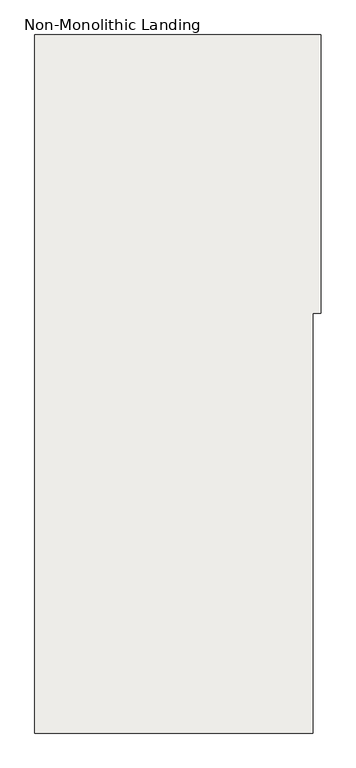
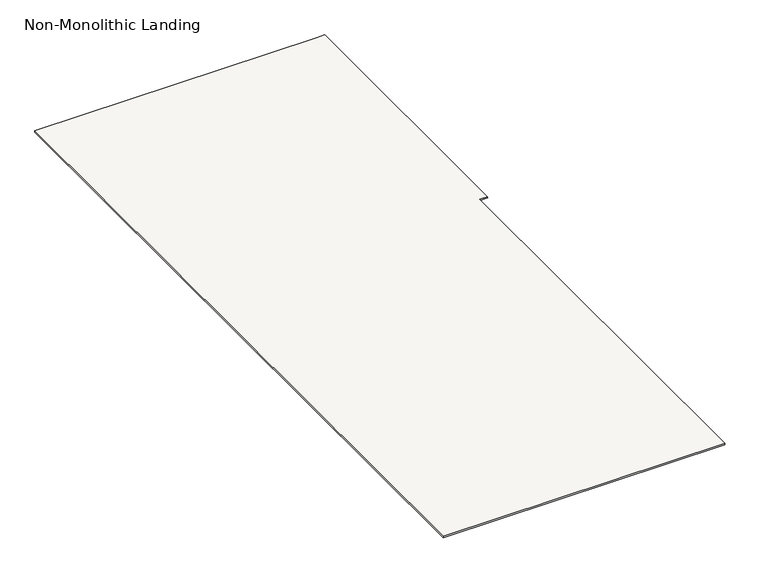
"""IFC4 building model written with IfcOpenShell, lengths in millimetres: slab geometry, Non-Monolithic Landing."""

from ifc_helpers import new_model, si_unit, origin, place, context, project, spatial, faceted_brep, source, transform, mapped, element, save


def non_monolithic_landing_6a719e3e(model_context):
    return source(origin(), model_context, "Body", "Brep", [
        faceted_brep([(-16318.9400908, 12030.4345331, 9941.1764706), (-16318.0900908, 12030.4345331, 9935.1764706), (-16318.0900908, 13130.4345331, 9935.1764706), (-16318.9400908, 13130.4345331, 9941.1764706), (-16350.0, 11470.4345331, 9941.1764706), (-16350.0, 12030.4345331, 9941.1764706), (-16350.0, 13130.4345331, 9941.1764706), (-17450.0, 13130.4345331, 9941.1764706), (-17450.0, 10370.4345331, 9941.1764706), (-16350.0, 10370.4345331, 9941.1764706), (-16350.0, 12030.4345331, 9935.1764706), (-16350.0, 11470.4345331, 9935.1764706), (-16350.85, 11470.4345331, 9935.1764706), (-16350.85, 10370.4345331, 9935.1764706), (-17450.0, 10370.4345331, 9935.1764706), (-17450.0, 13130.4345331, 9935.1764706), (-16350.0, 13130.4345331, 9935.1764706)], [[[0, 1, 2, 3]], [[4, 5, 0, 3, 6, 7, 8, 9]], [[10, 11, 12, 13, 14, 15, 16, 2, 1]], [[5, 4, 11, 10]], [[0, 5, 10, 1]], [[6, 3, 2, 16]], [[7, 6, 16, 15]], [[8, 7, 15, 14]], [[9, 8, 14, 13]], [[4, 12, 11]], [[12, 4, 9, 13]]]),
    ])


if __name__ == "__main__":
    model = new_model("IFC4")
    model_context = context("Model", 3, world=origin())
    ifc_project = project(units=[si_unit("LENGTHUNIT", "METRE", prefix="MILLI")], contexts=[model_context])
    site = spatial("IfcSite", under=ifc_project)
    building = spatial("IfcBuilding", under=site)
    placement = place(None, origin())
    non_monolithic_landing_shape = non_monolithic_landing_6a719e3e(model_context)
    element("IfcSlab", 1, ObjectType="Non-Monolithic Landing", at=placement, inside=building, context=model_context, shape_type="MappedRepresentation", body=[
        mapped(non_monolithic_landing_shape, transform((0.0, 0.0, 0.0), x_axis=(1.0, 0.0, 0.0), y_axis=(0.0, 1.0, 0.0), z_axis=(0.0, 0.0, 1.0))),
    ])
    save(model, "model.ifc")

# Revit data of these elements
# Element 1 (IfcSlab, "Non-Monolithic Landing")
#   Materials on its faces: "Steel, Paint Finish, Dark Gray"
# Materials
#   "Steel, Paint Finish, Dark Gray": class "Metal", colour RGB 89 89 89, transparency 0, Description = "Steel, paint finish, dark gray, glossy", Cost = 0
